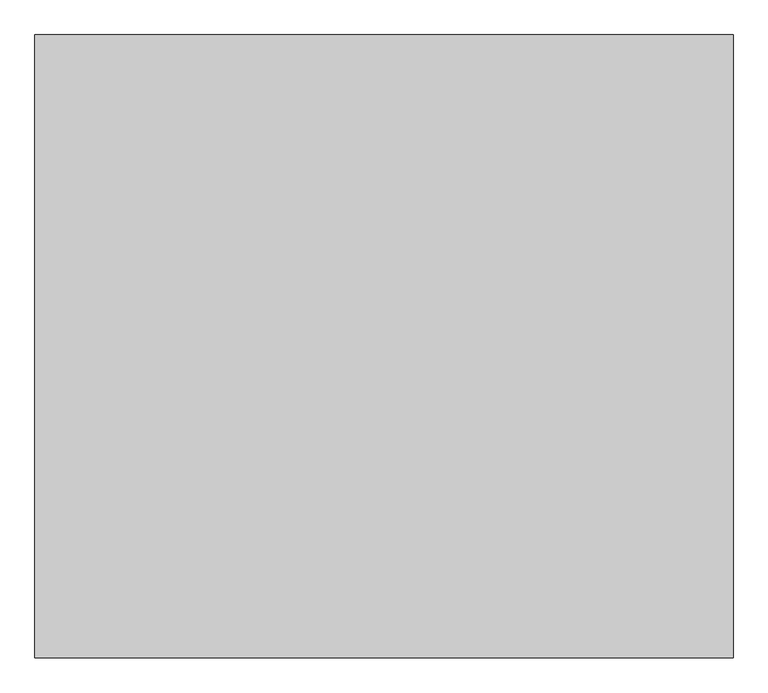
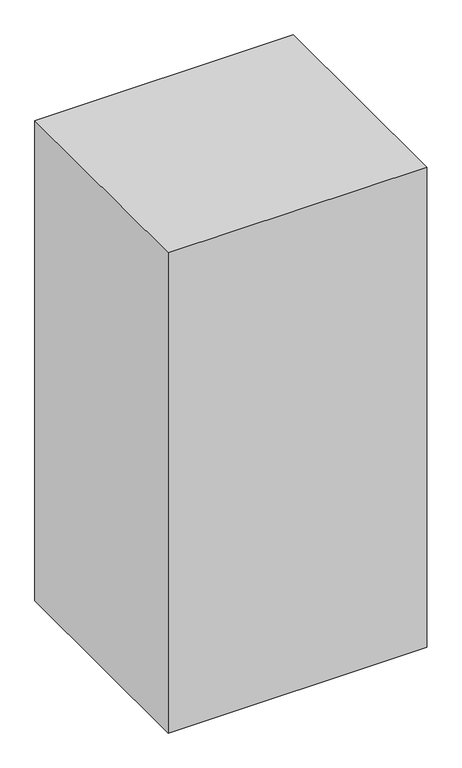
"""IFC4 building model written with IfcOpenShell, lengths in millimetres: proxy geometry, Space Planning Box_hec : Space Planning Box_hec."""

import ifcopenshell
import ifcopenshell.guid

model = None  # the IFC model being written
_history = None  # IfcOwnerHistory: only IFC2X3 demands one
_inside = {}  # id of a spatial element -> (the spatial element, [elements in it])
_under = {}  # id of a project, library or spatial element -> (it, [spatial elements below it])
_declared = {}  # id of a project -> (the project, [libraries it declares])
_typed = {}  # id of a type object -> (the type object, [elements of that type])
_made_of = {}  # id of a material, layer set ... -> (it, [elements and type objects made of it])


def new_model(schema):
    """Start an empty IFC model of exactly this schema.

    Asked for "IFC4X3", IfcOpenShell would pick the latest addendum, in which some entities
    have other attributes; the version numbers below select the first issue.
    IFC2X3 requires an IfcOwnerHistory on every rooted entity: one is made here for all.
    """
    global model, _history
    if schema == "IFC4X3":
        model = ifcopenshell.file(schema_version=(4, 3, 0, 0))
    else:
        model = ifcopenshell.file(schema=schema)
    _inside.clear()
    _under.clear()
    _declared.clear()
    _typed.clear()
    _made_of.clear()
    _history = None
    if model.schema == "IFC2X3":
        org = make("IfcOrganization", Name="unknown")
        user = make(
            "IfcPersonAndOrganization",
            ThePerson=make("IfcPerson", FamilyName="unknown"),
            TheOrganization=org,
        )
        app = make(
            "IfcApplication",
            ApplicationDeveloper=org,
            Version="unknown",
            ApplicationFullName="unknown",
            ApplicationIdentifier="unknown",
        )
        _history = make(
            "IfcOwnerHistory",
            OwningUser=user,
            OwningApplication=app,
            ChangeAction="ADDED",
            CreationDate=0,
        )
    return model


def make(cls, **values):
    """One entity of the class cls with the attributes given. An attribute that is None is left unset."""
    return model.create_entity(
        cls, **{name: value for name, value in values.items() if value is not None}
    )


def rooted(cls, **values):
    """An entity with a GlobalId (a new one), such as an element, a storey or a relation."""
    return make(cls, GlobalId=ifcopenshell.guid.new(), OwnerHistory=_history, **values)


def si_unit(unit_type, name, prefix=None):
    """IfcSIUnit, for example si_unit("LENGTHUNIT", "METRE", prefix="MILLI")."""
    return make("IfcSIUnit", UnitType=unit_type, Prefix=prefix, Name=name)


def assignment(units):
    """IfcUnitAssignment: the units of a project."""
    return None if units is None else make("IfcUnitAssignment", Units=units)


def point(xyz):
    """IfcCartesianPoint."""
    return None if xyz is None else make("IfcCartesianPoint", Coordinates=xyz)


def direction(xyz):
    """IfcDirection."""
    return None if xyz is None else make("IfcDirection", DirectionRatios=xyz)


def frame(location, z_axis=None, x_axis=None):
    """IfcAxis2Placement3D, a coordinate frame: its origin and axes. An axis left out is left unset."""
    return make(
        "IfcAxis2Placement3D",
        Location=point(location),
        Axis=direction(z_axis),
        RefDirection=direction(x_axis),
    )


def origin():
    """The frame at (0, 0, 0) with its axes left unset."""
    return frame((0.0, 0.0, 0.0))


def origin_with_axes():
    """The frame at (0, 0, 0) with the z axis (0, 0, 1) and the x axis (1, 0, 0) written out."""
    return frame((0.0, 0.0, 0.0), z_axis=(0.0, 0.0, 1.0), x_axis=(1.0, 0.0, 0.0))


def place(relative_to, where):
    """IfcLocalPlacement: puts the frame where relative to a parent placement (None: the world)."""
    return make(
        "IfcLocalPlacement", PlacementRelTo=relative_to, RelativePlacement=where
    )


def context(
    kind, dimensions, precision=None, world=None, true_north=None, identifier=None
):
    """IfcGeometricRepresentationContext, for example the 3D "Model" context."""
    return make(
        "IfcGeometricRepresentationContext",
        ContextIdentifier=identifier,
        ContextType=kind,
        CoordinateSpaceDimension=dimensions,
        Precision=precision,
        WorldCoordinateSystem=world,
        TrueNorth=true_north,
    )


def project(units=None, contexts=None):
    """IfcProject with its units and contexts."""
    return rooted(
        "IfcProject",
        Name="project",
        RepresentationContexts=contexts,
        UnitsInContext=assignment(units),
    )


def spatial(cls, under=None, at=None, **own):
    """A site, building, storey or space (cls), placed at a placement, below another one or the project."""
    s = rooted(cls, ObjectPlacement=at, **own)
    if under is not None:
        _under.setdefault(under.id(), (under, []))[1].append(s)
    return s


def polyline(points):
    """IfcPolyline through the points."""
    return make("IfcPolyline", Points=[point(p) for p in points])


def outline(outer, holes=None, kind="AREA"):
    """IfcArbitraryClosedProfileDef: a profile drawn as a closed curve; with holes, ...WithVoids."""
    if holes is None:
        return make("IfcArbitraryClosedProfileDef", ProfileType=kind, OuterCurve=outer)
    return make(
        "IfcArbitraryProfileDefWithVoids",
        ProfileType=kind,
        OuterCurve=outer,
        InnerCurves=holes,
    )


def extrude(swept, where, along, depth):
    """IfcExtrudedAreaSolid: the profile swept, set in the frame where, extruded along a direction by depth."""
    return make(
        "IfcExtrudedAreaSolid",
        SweptArea=swept,
        Position=where,
        ExtrudedDirection=direction(along),
        Depth=depth,
    )


def shape(context_of_items, identifier, shape_type, items):
    """IfcShapeRepresentation: the items that make up one representation, for example the "Body"."""
    return make(
        "IfcShapeRepresentation",
        ContextOfItems=context_of_items,
        RepresentationIdentifier=identifier,
        RepresentationType=shape_type,
        Items=items,
    )


def source(mapping_origin, context_of_items, identifier, shape_type, items):
    """IfcRepresentationMap: a shape defined once, which mapped items show again and again."""
    return make(
        "IfcRepresentationMap",
        MappingOrigin=mapping_origin,
        MappedRepresentation=shape(context_of_items, identifier, shape_type, items),
    )


def transform(
    local_origin,
    x_axis=None,
    y_axis=None,
    z_axis=None,
    scale=None,
    scale2=None,
    scale3=None,
    uniform=True,
):
    """IfcCartesianTransformationOperator3D, or its non-uniform kind. x_axis, y_axis, z_axis: its Axis1, 2, 3."""
    if uniform:
        return make(
            "IfcCartesianTransformationOperator3D",
            Axis1=direction(x_axis),
            Axis2=direction(y_axis),
            LocalOrigin=point(local_origin),
            Scale=scale,
            Axis3=direction(z_axis),
        )
    return make(
        "IfcCartesianTransformationOperator3DnonUniform",
        Axis1=direction(x_axis),
        Axis2=direction(y_axis),
        LocalOrigin=point(local_origin),
        Scale=scale,
        Axis3=direction(z_axis),
        Scale2=scale2,
        Scale3=scale3,
    )


def mapped(mapping_source, mapping_target):
    """IfcMappedItem: shows the shape of a source again, moved by a transform."""
    return make(
        "IfcMappedItem", MappingSource=mapping_source, MappingTarget=mapping_target
    )


def made_of(thing, what):
    """Note that an element or type object is made of a material, layer set ...; save() writes the relation."""
    if what is not None:
        _made_of.setdefault(what.id(), (what, []))[1].append(thing)
    return thing


def element(
    cls,
    number,
    at=None,
    inside=None,
    cuts=None,
    type_object=None,
    material=None,
    context=None,
    identifier="Body",
    shape_type=None,
    held_by="IfcProductDefinitionShape",
    body=None,
    shapes=None,
    **own,
):
    """One element of the class cls, such as IfcWall. Its Tag is "e" and its number.

    at: its placement. inside: the storey or other place that contains it. cuts: it is an
    opening in that element (IfcRelVoidsElement). A single representation is given by context,
    identifier, shape_type and body (its items); several are given by shapes. held_by: the class
    of the entity that holds the representations. save() writes the other relations.
    """
    e = rooted(cls, Tag="e%d" % number, ObjectPlacement=at, **own)
    if body is not None:
        shapes = [shape(context, identifier, shape_type, body)]
    if shapes is not None:
        e.Representation = make(held_by, Representations=shapes)
    if inside is not None:
        _inside.setdefault(inside.id(), (inside, []))[1].append(e)
    if cuts is not None:
        rooted(
            "IfcRelVoidsElement", RelatingBuildingElement=cuts, RelatedOpeningElement=e
        )
    if type_object is not None:
        _typed.setdefault(type_object.id(), (type_object, []))[1].append(e)
    return made_of(e, material)


def aggregate(whole, parts):
    """IfcRelAggregates: a whole, such as a stair, and the parts it consists of."""
    return rooted("IfcRelAggregates", RelatingObject=whole, RelatedObjects=parts)


def save(model, path):
    """Write the relations noted so far, then the file.

    IfcRelAggregates (storeys below a building ...), IfcRelContainedInSpatialStructure (elements
    in a storey), IfcRelDefinesByType, IfcRelAssociatesMaterial and IfcRelDeclares: one each for
    every whole, place, type object, material and project.
    """
    for whole, parts in _under.values():
        aggregate(whole, parts)
    for where, things in _inside.values():
        rooted(
            "IfcRelContainedInSpatialStructure",
            RelatedElements=things,
            RelatingStructure=where,
        )
    for kind, things in _typed.values():
        rooted("IfcRelDefinesByType", RelatedObjects=things, RelatingType=kind)
    for what, things in _made_of.values():
        rooted("IfcRelAssociatesMaterial", RelatedObjects=things, RelatingMaterial=what)
    for by, libraries in _declared.values():
        rooted("IfcRelDeclares", RelatingContext=by, RelatedDefinitions=libraries)
    model.write(path)


def generic_models_0ee3397c(model_context):
    return source(origin(), model_context, "Body", "SweptSolid", [
        extrude(outline(polyline([(1400.0, 1250.0), (1400.0, -1250.0), (-1400.0, -1250.0), (-1400.0, 1250.0), (1400.0, 1250.0)])), origin_with_axes(), (0.0, 0.0, 1.0), 5500.0),
    ])


if __name__ == "__main__":
    model = new_model("IFC4")
    model_context = context("Model", 3, world=origin())
    ifc_project = project(units=[si_unit("LENGTHUNIT", "METRE", prefix="MILLI")], contexts=[model_context])
    site = spatial("IfcSite", under=ifc_project)
    building = spatial("IfcBuilding", under=site)
    placement = place(None, origin())
    generic_models_shape = generic_models_0ee3397c(model_context)
    element("IfcBuildingElementProxy", 1, Name="Space Planning Box_hec : Space Planning Box_hec", ObjectType="Space Planning Box_hec : Space Planning Box_hec", at=placement, inside=building, context=model_context, shape_type="MappedRepresentation", body=[
        mapped(generic_models_shape, transform((0.0, 0.0, 0.0), x_axis=(1.0, 0.0, 0.0), y_axis=(0.0, 1.0, 0.0), z_axis=(0.0, 0.0, 1.0))),
    ])
    save(model, "model.ifc")

# Revit data of these elements
# Project information
#   Building Name = "MAIN GATE SECURITY BUILDING"
#   Project Status = "Project Status"
#   Client Name = "현대엔지니어링"
#   Project Address = "서울시 종로구 율곡로 75(계동)"
#   Project Name = "Therma Visayas Energy Project"
#   Project Number = "-"
# Type "Space Planning Box_hec : Space Planning Box_hec"
#   Type Comments = "..."
#   Room Name [instance default] = "?"
#   Interior Finish [instance default] = ""
#   Exterior Finish [instance default] = ""
#   Department [instance default] = ""
#   Assembly Code = "..."
#   Width [instance default] = 1524 mm
#   Program Area [instance default] = 0.00 m²
#   Length [instance default] = 1524 mm
#   Height [instance default] = 1524 mm
#   Area [instance default] = 2.32258 m²
#   Fill Color [instance default] = Cyan
#   Default Elevation = 0
# Element 1 (IfcBuildingElementProxy, "Space Planning Box_hec : Space Planning Box_hec")
#   Room Name = "Locker(F)"
#   Width = 2800 mm
#   Program Area = 7.00 m²
#   Length = 2500 mm
#   Height = 5500 mm
#   Area = 7.00 m²
#   Materials on its faces: "Cyan"
# Materials
#   "Cyan": class "Generic", colour RGB 0 255 255, transparency 0.2, Cost = 0
